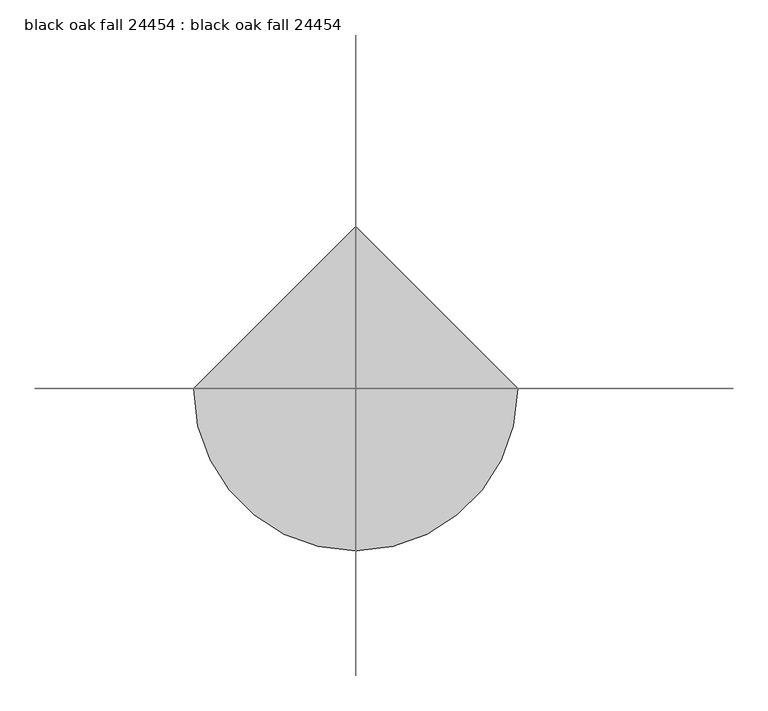
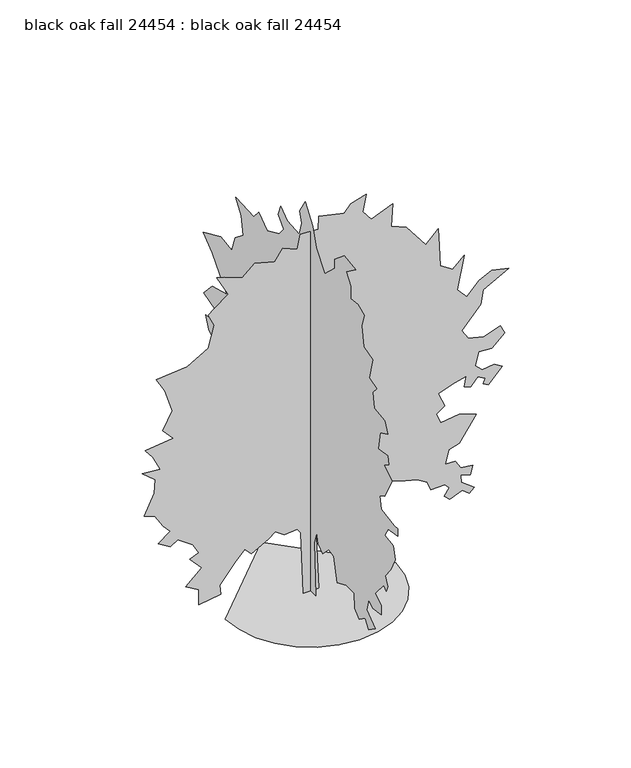
"""IFC4 building model written with IfcOpenShell, lengths in millimetres: proxy geometry, black oak fall 24454 : black oak fall 24454."""

from ifc_helpers import new_model, si_unit, origin, place, context, project, spatial, triangles, source, transform, mapped, element, save


def black_oak_fall_24454_black_oak_fall_24454_83d15e47(model_context):
    return source(origin(), model_context, "Body", "Tessellation", [
        triangles([(-3837.6128494, 0.0, 0.0005382), (-3736.1652626, -879.3283762, 0.0005382), (-3447.2145859, -1686.8483448, 0.0005382), (-2993.9256844, -2399.4281055, 0.0005382), (-2399.4281055, -2993.9256844, 0.0005382), (-1686.8483448, -3447.2145859, 0.0005382), (-879.3258327, -3736.1652626, 0.0005382), (0.0001677, -3837.6128494, 0.0005382), (879.3283762, -3736.1652626, 0.0005382), (1686.8483448, -3447.2145859, 0.0005382), (2399.4281055, -2993.9256844, 0.0005382), (2993.9256844, -2399.4281055, 0.0005382), (3447.2145859, -1686.8483448, 0.0005382), (3736.1652626, -879.3258327, 0.0005382), (3837.6128494, 0.0003355, 0.0005382), (-0.0005032, 3837.6128494, 0.0005382), (-323.0907804, 0.0, 0.0080165), (-450.6217678, -0.0001748, 2933.2197968), (-603.6594106, -0.000187, 3137.2835037), (-1190.3059061, -0.000184, 3086.2549324), (-1598.4054874, -0.0002007, 3366.8488518), (-1904.4808456, -0.000187, 3137.2835037), (-2669.6690231, -0.0001612, 2703.6797379), (-2975.7392944, -0.0001809, 3035.2516502), (-3409.3430603, -0.0001505, 2525.1278458), (-4098.0138153, -0.0001019, 1708.926067), (-4047.0105331, -7.45e-05, 1249.8131023), (-5041.7515594, -6.54e-05, 1096.7754232), (-5041.7515594, -0.0001079, 1810.9528336), (-5628.3907516, -0.0001292, 2168.0416477), (-4914.2180649, -0.0001688, 2831.2132324), (-5449.8539749, -0.0002037, 3417.8521339), (-5041.7515594, -0.0002128, 3570.8872696), (-5322.3204803, -0.0002417, 4055.4943176), (-5985.4893036, -0.0002706, 4540.1266548), (-6317.0615067, -0.0002569, 4310.5613068), (-6878.1987671, -0.0002767, 4642.1585083), (-6317.0615067, -0.000301, 5050.2609238), (-6648.6587082, -0.0003223, 5407.3338959), (-7031.2591919, -0.0003588, 6019.5000183), (-7490.3643082, -0.0003679, 6172.5348633), (-7056.7605423, -0.0004242, 7116.2726074), (-7005.7322617, -0.0004622, 7753.9150818), (-7592.3964523, -0.0004911, 8238.5471283), (-6776.1922028, -0.0004865, 8162.0169159), (-7107.7638245, -0.0005275, 8850.6876709), (-7464.8629578, -0.0005534, 9284.2914368), (-6189.5280121, -0.0005625, 9437.3268631), (-6674.1600586, -0.0005944, 9972.9621918), (-6240.5562927, -0.0006416, 10763.6650909), (-6572.1284958, -0.0007054, 11834.9357483), (-6954.7289795, -0.0007449, 12498.0801544), (-5551.8855377, -0.0007525, 12625.6130676), (-4608.1477936, -0.000786, 13186.7509094), (-4353.0808044, -0.0008453, 14181.5169342), (-4608.1477936, -0.0008787, 14742.654776), (-4353.0808044, -0.0008924, 14972.1942535), (-3715.4389114, -0.0009198, 15431.325531), (-4225.5473099, -0.0009776, 16400.5640442), (-3893.9753975, -0.0009715, 16298.5330627), (-3077.7711479, -0.0009532, 15992.4622101), (-2516.631562, -0.0009836, 16502.5706085), (-1623.9122154, -0.0009684, 16247.5036194), (-1266.8234013, -0.0010004, 16783.1395294), (-603.6594106, -0.0009836, 16502.5706085), (-476.1284595, -0.0010232, 17165.7405945), (340.0732467, -0.0010201, 17114.736731), (365.5799383, -0.0010566, 17726.8772736), (1513.3637306, -0.0010414, 17471.8102844), (1819.4364727, -0.0010612, 17803.407486), (2508.1096985, -0.0010748, 18032.9481262), (2355.0696213, -0.0010277, 17242.2708069), (2737.6648727, -0.0009988, 16757.6375977), (3706.904258, -0.0010216, 17140.2386627), (3630.3740456, -0.0009593, 16094.4687744), (4319.0448006, -0.0009426, 15813.8998535), (5186.2776215, -0.0008757, 14691.6253326), (5747.4148819, -0.0009091, 15252.7631744), (5798.4181641, -0.000859, 14411.0575745), (5849.4214462, -0.0008012, 13441.8178986), (6410.5842865, -0.0007799, 13084.7443451), (6920.6926849, -0.0008088, 13569.3508118), (6614.6224136, -0.0007176, 12038.9744568), (7048.2261795, -0.0006887, 11554.3679901), (7609.3634399, -0.0007237, 12141.006601), (8170.5007004, -0.0007404, 12421.5755219), (8935.7016678, -0.0007297, 12243.0387451), (7787.9002167, -0.0006933, 11630.8726227), (7660.3923019, -0.0006537, 10967.7037994), (6818.6611221, -0.000596, 9998.4641235), (7099.2550415, -0.0005701, 9564.8603577), (7813.4271469, -0.0005595, 9386.3235809), (8553.1011841, -0.0005747, 9641.3905701), (8757.1398926, -0.0005503, 9233.2881546), (8170.5007004, -0.0005184, 8697.6528259), (7583.8620895, -0.0005215, 8748.6561081), (7430.8266632, -0.000485, 8136.5155655), (7736.8969345, -0.0004667, 7830.4452942), (8272.5328445, -0.0004713, 7906.9499268), (8629.6313965, -0.0004576, 7677.4098679), (8017.4658554, -0.0004181, 7014.2410446), (7787.9002167, -0.0004257, 7141.7745392), (7864.4304291, -0.0004394, 7371.3145981), (7532.8588074, -0.0004515, 7575.3783051), (7226.7629562, -0.0004287, 7192.7778214), (6920.6926849, -0.0004348, 7294.8093842), (7022.7248291, -0.0004637, 7779.4164322), (6487.0889191, -0.0004561, 7651.8829376), (5747.4148819, -0.0004394, 7371.3145981), (6053.4851532, -0.0003998, 6708.1707733), (5670.8846695, -0.0003831, 6427.6018524), (5874.9483765, -0.0003542, 5942.9698059), (6691.152626, -0.0003618, 6070.5033005), (7456.328595, -0.0003466, 5815.4363113), (6691.152626, -0.0002797, 4693.1617905), (6232.0219299, -0.0002706, 4540.1266548), (6078.987085, -0.0002326, 3902.459182), (6512.5908508, -0.0002326, 3902.459182), (6767.65784, -0.0002083, 3494.3570572), (7303.2931686, -0.0002037, 3417.8521339), (7201.2616058, -0.0001794, 3009.7500092), (6767.65784, -0.000187, 3137.2835037), (6793.1591904, -0.0001672, 2805.6863022), (7379.823381, -0.0001399, 2346.583366), (7150.2583237, -0.0001277, 2142.5349197), (6844.1880524, -0.0001429, 2397.596822), (6283.0507919, -0.0001292, 2168.0416477), (6027.9838028, -0.0001429, 2397.596822), (6257.5238617, -0.0001627, 2729.1813789), (6053.4851532, -0.0001748, 2933.2197968), (5415.8176804, -0.0001748, 2933.2197968), (5262.7828354, -0.0001992, 3341.3219215), (4803.6771378, -0.0002159, 3621.8905518), (4268.0415184, -0.0002235, 3749.4240463), (3375.3326363, -0.0002402, 4029.9926765), (3120.2653564, -0.0002159, 3621.8905518), (2839.6970169, -0.0002311, 3876.9575409), (2712.1632317, -0.0002463, 4132.02453), (2202.0318695, -0.0002463, 4132.02453), (1946.9699673, -0.0002554, 4285.0596657), (1054.2481499, -0.0002417, 4055.4943176), (365.5799383, -0.0002159, 3621.8905518), (238.0474611, -0.0001764, 2958.746727), (365.5799383, 0.0, 0.0004815), (0.0, 369.5499722, 0.0), (0.0, 318.5391323, 2678.1528076), (0.0, 573.6010345, 3749.4240463), (0.0, 1032.7139992, 4336.0629478), (0.0, 1976.4466564, 4667.6601494), (0.0, 2563.0906448, 3902.459182), (0.0, 2767.1543518, 4336.0629478), (0.0, 3557.8316711, 4080.9959587), (0.0, 4118.9689316, 4157.5261711), (0.0, 4858.6682579, 3392.3252037), (0.0, 5496.3104416, 2601.6478844), (0.0, 6159.4792648, 2550.619313), (0.0, 5776.8787811, 3239.2900681), (0.0, 6644.1118927, 3519.8586983), (0.0, 6133.9779144, 3749.4240463), (0.0, 5241.2434525, 4157.5261711), (0.0, 5751.3774307, 4922.7268478), (0.0, 6236.0100586, 5509.36604), (0.0, 6031.9457703, 6198.036795), (0.0, 6440.0481857, 7039.742395), (0.0, 6924.6808136, 6810.1773376), (0.0, 7587.824057, 6580.6372787), (0.0, 8072.4566849, 6606.1386292), (0.0, 7511.3194244, 7371.3145981), (0.0, 7944.9231903, 7651.8829376), (0.0, 8174.488829, 8213.0201981), (0.0, 7511.3194244, 8238.5221298), (0.0, 7409.2872803, 8876.1896027), (0.0, 8327.523674, 9156.7579422), (0.0, 7664.3542694, 9870.9300476), (0.0, 6542.0797485, 10177.0009003), (0.0, 7664.3542694, 11477.8377777), (0.0, 8378.5269562, 12013.472525), (0.0, 7001.1854462, 12625.6130676), (0.0, 6159.4792648, 12498.0801544), (0.0, 5904.4122757, 13237.7791901), (0.0, 5241.2434525, 13773.3895203), (0.0, 5419.805809, 14589.5943512), (0.0, 5853.4089935, 15201.7593109), (0.0, 4425.064492, 15150.7310303), (0.0, 4067.9656494, 15584.360376), (0.0, 3404.7965355, 15099.7283295), (0.0, 2461.0689651, 15533.3320953), (0.0, 2103.980151, 15966.9358612), (0.0, 2512.079805, 16426.065976), (0.0, 2333.5354706, 16910.6736053), (0.0, 1823.4115208, 16528.0725403), (0.0, 905.1830481, 16451.5679077), (0.0, 675.6278738, 17114.736731), (0.0, 854.1696648, 17599.3443604), (0.0, 420.5633918, 18288.0151154), (0.0, -166.0810872, 17471.8102844), (0.0, -446.6491905, 16630.1046844), (0.0, -1109.8132175, 15788.3990845), (0.0, -1900.5082684, 16528.0725403), (0.0, -1875.0041565, 16936.1743744), (0.0, -2640.1798347, 17573.8424286), (0.0, -3507.4126556, 17420.8075836), (0.0, -2767.7133293, 16885.1716736), (0.0, -3124.8121719, 16400.5396271), (0.0, -3124.8121719, 15813.8998535), (0.0, -3685.9494324, 15890.4300659), (0.0, -4196.0834106, 15686.3669403), (0.0, -3992.0197037, 15048.7244659), (0.0, -4145.0548393, 14155.9905853), (0.0, -4833.7255943, 13951.9518768), (0.0, -4578.6838943, 12931.6839203), (0.0, -5165.3225052, 12753.1471436), (0.0, -4859.2525246, 12421.5755219), (0.0, -4961.2587982, 11707.4028351), (0.0, -5777.4630478, 11605.3706909), (0.0, -6007.0286865, 11095.2367126), (0.0, -5420.3894943, 10814.6677917), (0.0, -5292.8559998, 9972.9621918), (0.0, -6007.0286865, 10074.9943359), (0.0, -6109.0602493, 9717.8952026), (0.0, -5700.9584152, 9462.8282135), (0.0, -6364.10224, 9080.2533096), (0.0, -5777.4630478, 8008.9820709), (0.0, -5394.8625641, 7804.918364), (0.0, -5496.8947083, 7218.2791718), (0.0, -6542.6640152, 7065.2443268), (0.0, -6797.7310043, 7090.7456772), (0.0, -6797.7310043, 6733.6721237), (0.0, -6058.0319687, 6606.1386292), (0.0, -5802.9649796, 6172.5348633), (0.0, -6466.1338028, 6070.5033005), (0.0, -6593.6672974, 5483.8641083), (0.0, -6262.0956757, 4795.193644), (0.0, -5828.4919098, 4259.5580246), (0.0, -6032.5300369, 3851.4558998), (0.0, -5904.9965424, 3570.8872696), (0.0, -5726.4597656, 3749.4240463), (0.0, -5037.7890106, 2933.2197968), (0.0, -5522.3960587, 2627.1495255), (0.0, -5522.3960587, 2219.0474007), (0.0, -4833.7255943, 2091.5163769), (0.0, -4527.655323, 2321.0741673), (0.0, -4374.6201874, 1759.934436), (0.0, -5037.7890106, 1249.8080154), (0.0, -4527.655323, 892.7218174), (0.0, -4247.0866928, 1275.3147434), (0.0, -3787.9812859, 943.7326572), (0.0, -3456.3840843, 1275.3147434), (0.0, -3405.3808022, 1938.4787704), (0.0, -2793.2402596, 1963.9854984), (0.0, -2079.0526028, 1657.9101402), (0.0, -1823.9907005, 2754.68302), (0.0, -1415.8885757, 2805.6863022), (0.0, -944.0222471, 2346.5782791), (0.0, -599.6894131, 2601.6478844), (0.0, -472.1584256, 3060.7532913), (0.0, -293.6115296, 2499.6160309), (0.0, -395.6383507, 0.0026911)], [[15, 16, 1], [14, 15, 1], [14, 1, 2], [13, 14, 2], [13, 2, 3], [13, 3, 4], [12, 13, 4], [11, 12, 4], [11, 4, 5], [11, 5, 6], [11, 6, 7], [11, 7, 8], [11, 8, 9], [11, 9, 10], [43, 44, 45], [81, 82, 83], [86, 87, 88], [85, 86, 88], [58, 59, 60], [77, 78, 79], [46, 47, 48], [58, 60, 61], [70, 71, 72], [84, 85, 88], [73, 74, 75], [51, 52, 53], [36, 37, 38], [35, 36, 38], [31, 32, 33], [84, 88, 89], [113, 114, 115], [29, 30, 31], [123, 124, 125], [123, 125, 126], [135, 136, 137], [67, 68, 69], [99, 100, 101], [98, 99, 101], [112, 113, 115], [112, 115, 116], [143, 144, 17], [143, 17, 18], [27, 28, 29], [26, 27, 29], [40, 41, 42], [119, 120, 121], [119, 121, 122], [69, 70, 72], [26, 29, 31], [25, 26, 31], [84, 89, 90], [105, 106, 107], [104, 105, 107], [45, 46, 48], [127, 128, 129], [126, 127, 129], [123, 126, 129], [122, 123, 129], [122, 129, 130], [65, 66, 67], [92, 93, 94], [92, 94, 95], [92, 95, 96], [91, 92, 96], [101, 102, 103], [98, 101, 103], [98, 103, 104], [97, 98, 104], [97, 104, 107], [135, 137, 138], [63, 64, 65], [109, 110, 111], [142, 143, 18], [142, 18, 19], [22, 23, 24], [119, 122, 130], [118, 119, 130], [117, 118, 130], [117, 130, 131], [117, 131, 132], [55, 56, 57], [48, 49, 50], [50, 51, 53], [25, 31, 33], [24, 25, 33], [117, 132, 133], [116, 117, 133], [112, 116, 133], [112, 133, 134], [112, 134, 135], [111, 112, 135], [77, 79, 80], [61, 62, 63], [111, 135, 138], [55, 57, 58], [83, 84, 90], [109, 111, 138], [109, 138, 139], [109, 139, 140], [80, 81, 83], [24, 33, 34], [91, 96, 97], [91, 97, 107], [91, 107, 108], [91, 108, 109], [90, 91, 109], [19, 20, 21], [142, 19, 21], [50, 53, 54], [69, 72, 73], [67, 69, 73], [65, 67, 73], [65, 73, 75], [48, 50, 54], [21, 22, 24], [21, 24, 34], [58, 61, 63], [55, 58, 63], [54, 55, 63], [54, 63, 65], [54, 65, 75], [48, 54, 75], [48, 75, 76], [48, 76, 77], [48, 77, 80], [48, 80, 83], [48, 83, 90], [48, 90, 109], [48, 109, 140], [48, 140, 141], [48, 141, 142], [48, 142, 21], [48, 21, 34], [45, 48, 34], [45, 34, 35], [45, 35, 38], [45, 38, 39], [45, 39, 40], [45, 40, 42], [45, 42, 43], [157, 158, 159], [201, 202, 203], [182, 183, 184], [155, 156, 157], [166, 167, 168], [200, 201, 203], [176, 177, 178], [154, 155, 157], [149, 150, 151], [172, 173, 174], [211, 212, 213], [165, 166, 168], [194, 195, 196], [193, 194, 196], [235, 236, 237], [169, 170, 171], [243, 244, 245], [243, 245, 246], [189, 190, 191], [188, 189, 191], [157, 159, 160], [154, 157, 160], [153, 154, 160], [250, 251, 252], [234, 235, 237], [199, 200, 203], [226, 227, 228], [226, 228, 229], [225, 226, 229], [193, 196, 197], [192, 193, 197], [168, 169, 171], [258, 145, 146], [257, 258, 146], [172, 174, 175], [221, 222, 223], [215, 216, 217], [214, 215, 217], [256, 257, 146], [256, 146, 147], [209, 210, 211], [184, 185, 186], [206, 207, 208], [218, 219, 220], [218, 220, 221], [246, 247, 248], [246, 248, 249], [243, 246, 249], [242, 243, 249], [253, 254, 255], [253, 255, 256], [239, 240, 241], [238, 239, 241], [238, 241, 242], [205, 206, 208], [199, 203, 204], [199, 204, 205], [198, 199, 205], [225, 229, 230], [181, 182, 184], [175, 176, 178], [175, 178, 179], [164, 165, 168], [164, 168, 171], [230, 231, 232], [230, 232, 233], [188, 191, 192], [221, 223, 224], [181, 184, 186], [192, 197, 198], [230, 233, 234], [153, 160, 161], [161, 162, 163], [153, 161, 163], [164, 171, 172], [164, 172, 175], [218, 221, 224], [198, 205, 208], [198, 208, 209], [198, 209, 211], [188, 192, 198], [187, 188, 198], [187, 198, 211], [186, 187, 211], [181, 186, 211], [181, 211, 213], [181, 213, 214], [181, 214, 217], [181, 217, 218], [181, 218, 224], [180, 181, 224], [179, 180, 224], [175, 179, 224], [164, 175, 224], [163, 164, 224], [153, 163, 224], [152, 153, 224], [151, 152, 224], [149, 151, 224], [148, 149, 224], [148, 224, 225], [147, 148, 225], [256, 147, 225], [253, 256, 225], [252, 253, 225], [252, 225, 230], [252, 230, 234], [252, 234, 237], [252, 237, 238], [250, 252, 238], [249, 250, 238], [242, 249, 238]], closed=False),
    ])


if __name__ == "__main__":
    model = new_model("IFC4")
    model_context = context("Model", 3, world=origin())
    ifc_project = project(units=[si_unit("LENGTHUNIT", "METRE", prefix="MILLI")], contexts=[model_context])
    site = spatial("IfcSite", under=ifc_project)
    building = spatial("IfcBuilding", under=site)
    placement = place(None, origin())
    black_oak_fall_24454_black_oak_fall_24454_shape = black_oak_fall_24454_black_oak_fall_24454_83d15e47(model_context)
    element("IfcBuildingElementProxy", 1, Name="black oak fall 24454 : black oak fall 24454", ObjectType="black oak fall 24454 : black oak fall 24454", at=placement, inside=building, context=model_context, shape_type="MappedRepresentation", body=[
        mapped(black_oak_fall_24454_black_oak_fall_24454_shape, transform((0.0, 0.0, 0.0), x_axis=(1.0, 0.0, 0.0), y_axis=(0.0, 1.0, 0.0), z_axis=(0.0, 0.0, 1.0))),
    ])
    save(model, "model.ifc")

# Revit data of these elements
# Type "black oak fall 24454 : black oak fall 24454"
#   built-in parameter 1005195 = "RPC-16-FX7S-WR7X-W9EP-G000-ST1L-LVER-AU"
#   Height = 0
